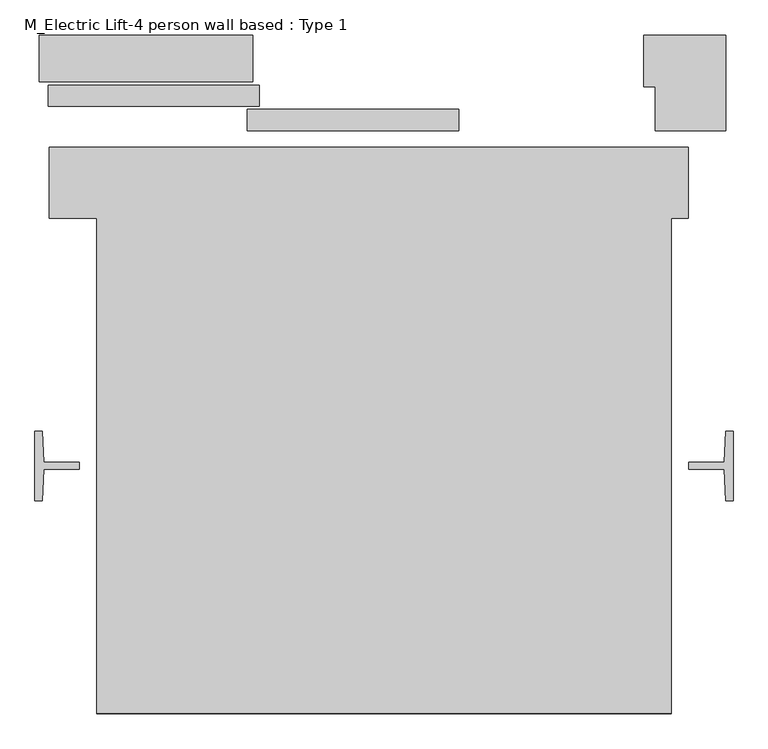
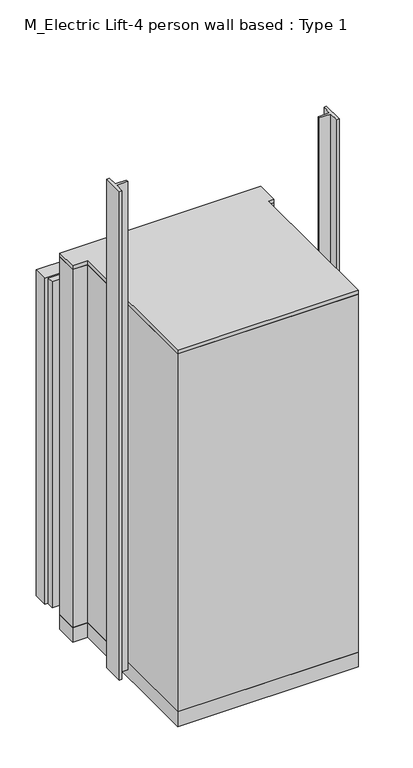
"""IFC4 building model written with IfcOpenShell, lengths in millimetres: proxy geometry, M_Electric Lift-4 person wall based : Type 1."""

from ifc_helpers import new_model, si_unit, frame, origin, origin_with_axes, place, context, project, spatial, polyline, outline, extrude, faceted_brep, source, transform, mapped, element, save


def m_electric_lift_4_person_wall_based_type_1_25105fba(model_context):
    return source(origin(), model_context, "Body", "SolidModel", [
        extrude(outline(polyline([(-400.0, -1140.0000001), (-400.0, -235.0), (-486.5, -235.0), (-486.5, -105.0), (681.0, -105.0), (681.0, -235.0), (650.0, -235.0), (650.0, -1140.0000001), (-400.0, -1140.0000001)])), frame((0.0, 0.0, 2200.0), z_axis=(0.0, 0.0, 1.0), x_axis=(1.0, 0.0, 0.0)), (0.0, 0.0, 1.0), 22.0),
        extrude(outline(polyline([(-448.6220553, -190.9893804), (-448.6220553, -149.3893804), (-62.6220553, -149.3893804), (-62.6220553, -190.9893804), (-448.6220553, -190.9893804)])), origin_with_axes(), (0.0, 0.0, 1.0), 2000.0),
        extrude(outline(polyline([(-114.8301, -144.0), (-114.8301, -108.9587126), (271.1699, -108.9587126), (271.1699, -144.0), (-114.8301, -144.0)])), origin_with_axes(), (0.0, 0.0, 1.0), 2000.0),
        extrude(outline(polyline([(-488.6220553, 8.3893803), (-102.6220553, 8.3893803), (-102.6220553, -30.6106197), (-488.6220553, -30.6106197), (-488.6220553, 8.3893803)])), origin_with_axes(), (0.0, 0.0, 1.0), 2000.0),
        extrude(outline(polyline([(-124.8301, -75.0), (-124.8301, -36.0), (261.1699, -36.0), (261.1699, -75.0), (-124.8301, -75.0)])), origin_with_axes(), (0.0, 0.0, 1.0), 2000.0),
        extrude(outline(polyline([(-400.0, -1140.0000001), (-400.0, -235.0), (-486.5, -235.0), (-486.5, -105.0), (681.0, -105.0), (681.0, -235.0), (650.0, -235.0), (650.0, -1140.0000001), (-400.0, -1140.0000001)])), frame((0.0, 0.0, -90.0), z_axis=(0.0, 0.0, 1.0), x_axis=(1.0, 0.0, 0.0)), (0.0, 0.0, 1.0), 90.0),
        faceted_brep([(-400.0, -1140.0000001, 2200.0), (650.0, -1140.0000001, 2200.0), (650.0, -235.0, 2200.0), (681.0, -235.0, 2200.0), (681.0, -105.0, 2200.0), (-486.5, -105.0, 2200.0), (-486.5, -235.0, 2200.0), (-400.0, -235.0, 2200.0), (-375.0, -1115.0000001, 2200.0), (-375.0, -235.0, 2200.0), (-110.3, -235.0, 2200.0), (-110.3, -197.0, 2200.0), (-458.1228936, -197.0, 2200.0), (-458.1228936, -108.9587126, 2200.0), (621.1699, -108.9587126, 2200.0), (621.1699, -192.6835257, 2200.0), (600.0, -192.6835257, 2200.0), (600.0, -235.0, 2200.0), (625.0, -235.0, 2200.0), (625.0, -572.5016433, 2200.0), (610.2454439, -572.5016433, 2200.0), (610.2454439, -802.5016433, 2200.0), (625.0, -802.5016433, 2200.0), (625.0, -1115.0000001, 2200.0), (-400.0, -1140.0000001, 0.0), (-400.0, -235.0, 0.0), (-486.5, -235.0, 0.0), (-486.5, -105.0, 0.0), (-173.4437103, -105.0, 0.0), (-173.4437103, -108.9587126, 0.0), (-458.1228936, -108.9587126, 0.0), (-458.1228936, -197.0, 0.0), (-110.3, -197.0, 0.0), (-110.3, -235.0, 0.0), (-375.0, -235.0, 0.0), (-375.0, -1115.0000001, 0.0), (625.0, -1115.0000001, 0.0), (625.0, -802.5016433, 0.0), (610.2454439, -802.5016433, 0.0), (610.2454439, -572.5016433, 0.0), (625.0, -572.5016433, 0.0), (625.0, -235.0, 0.0), (600.0, -235.0, 0.0), (600.0, -192.6835257, 0.0), (621.1699, -192.6835257, 0.0), (621.1699, -105.0, 0.0), (681.0, -105.0, 0.0), (681.0, -235.0, 0.0), (650.0, -235.0, 0.0), (650.0, -1140.0000001, 0.0), (621.1699, -105.0, 2000.0), (-173.4437103, -105.0, 2000.0), (-173.4437103, -108.9587126, 2000.0), (621.1699, -108.9587126, 2000.0), (600.0, -192.6835257, 2000.0)], [[[0, 1, 2, 3, 4, 5, 6, 7], [8, 9, 10, 11, 12, 13, 14, 15, 16, 17, 18, 19, 20, 21, 22, 23]], [[24, 25, 26, 27, 28, 29, 30, 31, 32, 33, 34, 35, 36, 37, 38, 39, 40, 41, 42, 43, 44, 45, 46, 47, 48, 49]], [[1, 0, 24, 49]], [[2, 1, 49, 48]], [[3, 2, 48, 47]], [[4, 3, 47, 46]], [[5, 4, 46, 45, 50, 51, 28, 27]], [[6, 5, 27, 26]], [[7, 6, 26, 25]], [[0, 7, 25, 24]], [[9, 8, 35, 34]], [[10, 9, 34, 33]], [[11, 10, 33, 32]], [[12, 11, 32, 31]], [[13, 12, 31, 30]], [[14, 13, 30, 29, 52, 53]], [[15, 14, 53, 50, 45, 44]], [[16, 15, 44, 43, 54]], [[17, 16, 54, 43, 42]], [[18, 17, 42, 41]], [[19, 18, 41, 40]], [[20, 19, 40, 39]], [[21, 20, 39, 38]], [[22, 21, 38, 37]], [[23, 22, 37, 36]], [[8, 23, 36, 35]], [[50, 53, 52, 51]], [[51, 52, 29, 28]]]),
        extrude(outline(polyline([(750.026988, -751.0012199), (747.026988, -693.80122), (682.0269884, -693.80122), (682.0269884, -681.3056039), (747.1132057, -681.3056039), (750.026988, -624.0012199), (763.026988, -624.0012199), (763.026988, -751.0012199), (750.026988, -751.0012199)])), origin_with_axes(), (0.0, 0.0, 1.0), 3000.0),
        extrude(outline(polyline([(-497.026988, -693.80122), (-500.026988, -751.0012199), (-513.026988, -751.0012199), (-513.026988, -624.0012199), (-500.026988, -624.0012199), (-497.1132057, -681.3056039), (-432.0269884, -681.3056039), (-432.0269884, -693.80122), (-497.026988, -693.80122)])), origin_with_axes(), (0.0, 0.0, 1.0), 3000.0),
        extrude(outline(polyline([(-114.9791786, 100.0), (-114.9791786, 14.4785696), (-505.0067971, 14.4785696), (-505.0067971, 100.0), (-114.9791786, 100.0)])), origin_with_axes(), (0.0, 0.0, 1.0), 2000.0),
        extrude(outline(polyline([(600.0, 5.0), (600.0, 100.0), (750.0, 100.0), (750.0, -75.0), (621.1699, -75.0), (621.1699, 5.0), (600.0, 5.0)])), origin_with_axes(), (0.0, 0.0, 1.0), 2000.0),
    ])


if __name__ == "__main__":
    model = new_model("IFC4")
    model_context = context("Model", 3, world=origin())
    ifc_project = project(units=[si_unit("LENGTHUNIT", "METRE", prefix="MILLI")], contexts=[model_context])
    site = spatial("IfcSite", under=ifc_project)
    building = spatial("IfcBuilding", under=site)
    placement = place(None, origin())
    m_electric_lift_4_person_wall_based_type_1_shape = m_electric_lift_4_person_wall_based_type_1_25105fba(model_context)
    element("IfcBuildingElementProxy", 1, Name="M_Electric Lift-4 person wall based : Type 1", ObjectType="M_Electric Lift-4 person wall based : Type 1", at=placement, inside=building, context=model_context, shape_type="MappedRepresentation", body=[
        mapped(m_electric_lift_4_person_wall_based_type_1_shape, transform((0.0, 0.0, 0.0), x_axis=(1.0, 0.0, 0.0), y_axis=(0.0, 1.0, 0.0), z_axis=(0.0, 0.0, 1.0))),
    ])
    save(model, "model.ifc")

# Revit data of these elements
# Type "M_Electric Lift-4 person wall based : Type 1"
#   Door Material = none
#   Manufacturer = ""
#   Default Elevation = 0
#   Assembly Code = ""
